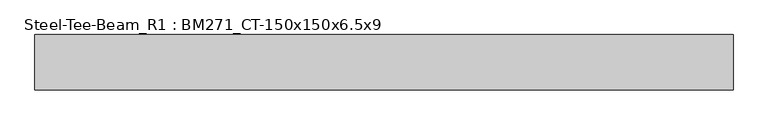
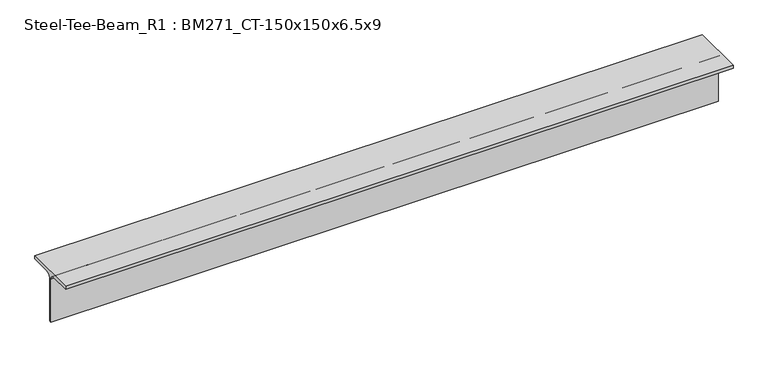
"""IFC4 building model written with IfcOpenShell, lengths in millimetres: member geometry, Steel-Tee-Beam_R1 : BM271_CT-150x150x6.5x9."""

from ifc_helpers import new_model, si_unit, point, frame, frame_2d, origin, place, context, project, spatial, polyline, circle_curve, trimmed, segment, composite_curve, outline, extrude, source, transform, mapped, element, save


def steel_tee_beam_r1_bm271_ct_150x150x6_5x9_075bac30(model_context):
    return source(origin(), model_context, "Body", "SweptSolid", [
        extrude(outline(composite_curve([segment(polyline([(75.0, 75.0), (75.0, 66.0), (16.25, 66.0)]), True, "CONTINUOUS"), segment(trimmed(circle_curve(frame_2d((16.25, 53.0)), 13.0), [point((16.25, 66.0))], [point((3.25, 53.0))], True, "CARTESIAN"), True, "CONTINUOUS"), segment(polyline([(3.25, 53.0), (3.25, -75.0), (-3.25, -75.0), (-3.25, 53.0)]), True, "CONTINUOUS"), segment(trimmed(circle_curve(frame_2d((-16.25, 53.0)), 13.0), [point((-3.25, 53.0))], [point((-16.25, 66.0))], True, "CARTESIAN"), True, "CONTINUOUS"), segment(polyline([(-16.25, 66.0), (-75.0, 66.0), (-75.0, 75.0), (75.0, 75.0)]), True, "CONTINUOUS")], self_intersect=False)), frame((-983.9814396, 0.0, 0.0), z_axis=(1.0, 0.0, 0.0), x_axis=(0.0, 1.0, 0.0)), (0.0, 0.0, 1.0), 1884.11033),
    ])


if __name__ == "__main__":
    model = new_model("IFC4")
    model_context = context("Model", 3, world=origin())
    ifc_project = project(units=[si_unit("LENGTHUNIT", "METRE", prefix="MILLI")], contexts=[model_context])
    site = spatial("IfcSite", under=ifc_project)
    building = spatial("IfcBuilding", under=site)
    placement = place(None, origin())
    steel_tee_beam_r1_bm271_ct_150x150x6_5x9_shape = steel_tee_beam_r1_bm271_ct_150x150x6_5x9_075bac30(model_context)
    element("IfcMember", 1, ObjectType="Steel-Tee-Beam_R1 : BM271_CT-150x150x6.5x9", at=placement, inside=building, context=model_context, shape_type="MappedRepresentation", body=[
        mapped(steel_tee_beam_r1_bm271_ct_150x150x6_5x9_shape, transform((0.0, 0.0, 0.0), x_axis=(1.0, 0.0, 0.0), y_axis=(0.0, 1.0, 0.0), z_axis=(0.0, 0.0, 1.0))),
    ])
    save(model, "model.ifc")

# Revit data of these elements
# Type "Steel-Tee-Beam_R1 : BM271_CT-150x150x6.5x9"
#   Keynote = "CT-150x150x6.5x9"
#   Surface Area = 0.588841 m²/m
#   Section Area = 23.3904 cm²
#   Mass per Unit Length = 18.3614 kg/m
#   Length [instance default] = 1.5240 m
#   bf = 0.1500 m
#   d = 0.1500 m
#   k = 0.0220 m
#   r = 0.0130 m
#   tf = 0.0090 m
#   tw = 0.0065 m
#   hec_material4 [instance default] = none
#   hec_material3 [instance default] = none
#   hec_material2 [instance default] = none
#   hec_material1 [instance default] = none
#   Structural Material [instance default] = Steel, 45-345
#   Assembly Code = ""
# Element 1 (IfcMember, "Steel-Tee-Beam_R1 : BM271_CT-150x150x6.5x9")
#   Structural Material = none
# Materials
#   "Steel, 45-345": class "Metal", colour RGB 189 187 185, transparency 0, Description = "Steel 345 MPa", Cost = 0
